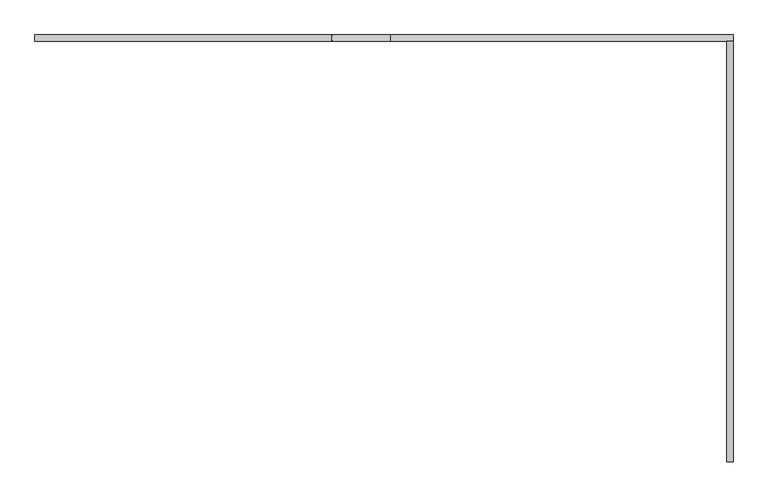
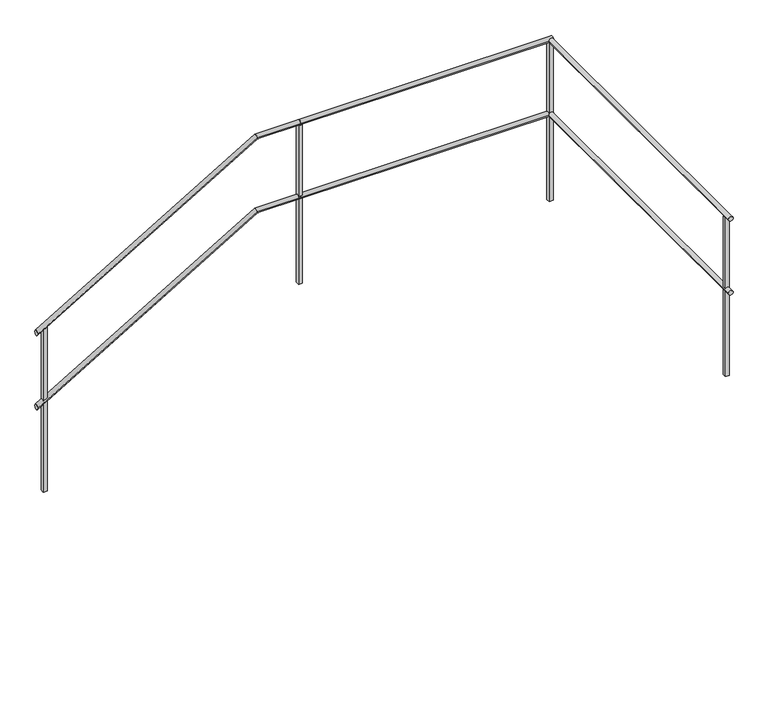
"""IFC4 building model written with IfcOpenShell, lengths in millimetres: railing geometry."""

from ifc_helpers import new_model, si_unit, frame, origin, place, context, project, spatial, polyline, circle_curve, ellipse_curve, outline, extrude, source, transform, mapped, element, save
from ifc_brep_helpers import plane_surface, cylinder_surface, advanced_brep


def railing_70c1d9d7(model_context):
    return source(origin(), model_context, "Body", "SolidModel", [
        advanced_brep(
        [(45466.7161135, 23749.5208589, 1584.9618634), (45496.7161135, 23749.5208589, 1584.9618634), (45466.7161135, 25734.1208589, 1584.9618634), (45496.7161135, 25734.1208589, 1584.9618634)],
        [
            (0, 1, circle_curve(frame((45481.7161135, 23749.5208589, 1584.9618634), z_axis=(0.0, -1.0, 0.0), x_axis=(1.0, 0.0, 0.0)), 15.0)),
            (1, 0, circle_curve(frame((45481.7161135, 23749.5208589, 1584.9618634), z_axis=(0.0, -1.0, 0.0), x_axis=(1.0, 0.0, 0.0)), 15.0)),
            (2, 3, circle_curve(frame((45481.7161135, 25734.1208589, 1584.9618634), z_axis=(0.0, 1.0, 0.0), x_axis=(1.0, 0.0, 0.0)), 15.0)),
            (3, 2, circle_curve(frame((45481.7161135, 25734.1208589, 1584.9618634), z_axis=(0.0, 1.0, 0.0), x_axis=(1.0, 0.0, 0.0)), 15.0)),
            (0, 2),
            (3, 1),
        ],
        [
            plane_surface(frame((45481.7161135, 23749.5208589, 1599.9618634), z_axis=(0.0, -1.0, 0.0), x_axis=(0.0, 0.0, 1.0))),
            plane_surface(frame((45481.7161135, 25734.1208589, 1599.9618634), z_axis=(0.0, 1.0, 0.0), x_axis=(0.0, 0.0, 1.0))),
            cylinder_surface(frame((45481.7161135, 23749.5208589, 1584.9618634), z_axis=(0.0, -1.0, 0.0), x_axis=(1.0, 0.0, 0.0)), 15.0),
        ],
        [
            (0, [[1, 2]]),
            (1, [[3, 4]]),
            (2, [[-1, 5, -4, 6]]),
            (2, [[-2, -6, -3, -5]]),
        ],
    ),
        advanced_brep(
        [(45496.7161135, 25734.1208589, 1584.9618634), (45496.7161135, 25764.1208589, 1584.9618634), (43882.1161135, 25734.1208589, 1584.9618634), (43882.1161135, 25764.1208589, 1584.9618634)],
        [
            (0, 1, circle_curve(frame((45496.7161135, 25749.1208589, 1584.9618634), z_axis=(1.0, 0.0, 0.0), x_axis=(0.0, 1.0, 0.0)), 15.0)),
            (1, 0, circle_curve(frame((45496.7161135, 25749.1208589, 1584.9618634), z_axis=(1.0, 0.0, 0.0), x_axis=(0.0, 1.0, 0.0)), 15.0)),
            (2, 3, circle_curve(frame((43882.1161135, 25749.1208589, 1584.9618634), z_axis=(-1.0, 0.0, 0.0), x_axis=(0.0, 1.0, 0.0)), 15.0)),
            (3, 2, circle_curve(frame((43882.1161135, 25749.1208589, 1584.9618634), z_axis=(-1.0, 0.0, 0.0), x_axis=(0.0, 1.0, 0.0)), 15.0)),
            (0, 2),
            (3, 1),
        ],
        [
            plane_surface(frame((45496.7161135, 25749.1208589, 1599.9618634), z_axis=(1.0, 0.0, 0.0), x_axis=(0.0, -1.0, 0.0))),
            plane_surface(frame((43882.1161135, 25749.1208589, 1599.9618634), z_axis=(-1.0, 0.0, 0.0), x_axis=(0.0, -1.0, 0.0))),
            cylinder_surface(frame((45496.7161135, 25749.1208589, 1584.9618634), z_axis=(1.0, 0.0, 0.0), x_axis=(0.0, 1.0, 0.0)), 15.0),
        ],
        [
            (0, [[1, 2]]),
            (1, [[3, 4]]),
            (2, [[-1, 5, -4, 6]]),
            (2, [[-2, -6, -3, -5]]),
        ],
    ),
        advanced_brep(
        [(43882.1161135, 25734.1208589, 1584.9618634), (43882.1161135, 25764.1208589, 1584.9618634), (43606.242552, 25734.1208589, 1584.9618634), (43606.242552, 25764.1208589, 1584.9618634), (42202.1161135, 25734.1208589, 749.1723166), (42202.1161135, 25764.1208589, 749.1723166)],
        [
            (0, 1, circle_curve(frame((43882.1161135, 25749.1208589, 1584.9618634), z_axis=(1.0, 0.0, 0.0), x_axis=(0.0, 1.0, 0.0)), 15.0)),
            (1, 0, circle_curve(frame((43882.1161135, 25749.1208589, 1584.9618634), z_axis=(1.0, 0.0, 0.0), x_axis=(0.0, 1.0, 0.0)), 15.0)),
            (0, 2),
            (2, 3, ellipse_curve(frame((43606.242552, 25749.1208589, 1584.9618634), z_axis=(0.9641817474962143, 0.0, 0.2652424509673111), x_axis=(0.265242450967311, 0.0, -0.9641817474962144)), 15.5572329, 15.0)),
            (3, 1),
            (3, 2, ellipse_curve(frame((43606.242552, 25749.1208589, 1584.9618634), z_axis=(0.9641817474962143, 0.0, 0.2652424509673111), x_axis=(0.265242450967311, 0.0, -0.9641817474962144)), 15.5572329, 15.0)),
            (4, 5, ellipse_curve(frame((42202.1161135, 25749.1208589, 749.1723166), z_axis=(-1.0, 0.0, 0.0), x_axis=(0.0, 0.0, 1.0)), 17.4562134, 15.0)),
            (5, 4, ellipse_curve(frame((42202.1161135, 25749.1208589, 749.1723166), z_axis=(-1.0, 0.0, 0.0), x_axis=(0.0, 0.0, 1.0)), 17.4562134, 15.0)),
            (2, 4),
            (5, 3),
        ],
        [
            plane_surface(frame((43882.1161135, 25749.1208589, 1599.9618634), z_axis=(1.0, 0.0, 0.0), x_axis=(0.0, -1.0, 0.0))),
            cylinder_surface(frame((43882.1161135, 25749.1208589, 1584.9618634), z_axis=(1.0, 0.0, 0.0), x_axis=(0.0, 1.0, 0.0)), 15.0),
            plane_surface(frame((42202.1161135, 25749.1208589, 766.62853), z_axis=(-1.0, 0.0, 0.0), x_axis=(0.0, -1.0, 0.0))),
            cylinder_surface(frame((43609.7883714, 25749.1208589, 1587.0724701), z_axis=(0.8592928844097072, 0.0, 0.5114838597676818), x_axis=(0.0, 1.0, 0.0)), 15.0),
        ],
        [
            (0, [[1, 2]]),
            (1, [[-1, 3, 4, 5]]),
            (1, [[-2, -5, 6, -3]]),
            (2, [[7, 8]]),
            (3, [[-4, 9, -8, 10]]),
            (3, [[-6, -10, -7, -9]]),
        ],
    ),
        advanced_brep(
        [(45466.7161135, 23749.5208589, 2084.9618634), (45496.7161135, 23749.5208589, 2084.9618634), (45466.7161135, 25734.1208589, 2084.9618634), (45496.7161135, 25734.1208589, 2084.9618634)],
        [
            (0, 1, circle_curve(frame((45481.7161135, 23749.5208589, 2084.9618634), z_axis=(0.0, -1.0, 0.0), x_axis=(1.0, 0.0, 0.0)), 15.0)),
            (1, 0, circle_curve(frame((45481.7161135, 23749.5208589, 2084.9618634), z_axis=(0.0, -1.0, 0.0), x_axis=(1.0, 0.0, 0.0)), 15.0)),
            (2, 3, circle_curve(frame((45481.7161135, 25734.1208589, 2084.9618634), z_axis=(0.0, 1.0, 0.0), x_axis=(1.0, 0.0, 0.0)), 15.0)),
            (3, 2, circle_curve(frame((45481.7161135, 25734.1208589, 2084.9618634), z_axis=(0.0, 1.0, 0.0), x_axis=(1.0, 0.0, 0.0)), 15.0)),
            (0, 2),
            (3, 1),
        ],
        [
            plane_surface(frame((45481.7161135, 23749.5208589, 2099.9618634), z_axis=(0.0, -1.0, 0.0), x_axis=(0.0, 0.0, 1.0))),
            plane_surface(frame((45481.7161135, 25734.1208589, 2099.9618634), z_axis=(0.0, 1.0, 0.0), x_axis=(0.0, 0.0, 1.0))),
            cylinder_surface(frame((45481.7161135, 23749.5208589, 2084.9618634), z_axis=(0.0, -1.0, 0.0), x_axis=(1.0, 0.0, 0.0)), 15.0),
        ],
        [
            (0, [[1, 2]]),
            (1, [[3, 4]]),
            (2, [[-1, 5, -4, 6]]),
            (2, [[-2, -6, -3, -5]]),
        ],
    ),
        advanced_brep(
        [(45496.7161135, 25734.1208589, 2084.9618634), (45496.7161135, 25764.1208589, 2084.9618634), (43882.1161135, 25734.1208589, 2084.9618634), (43882.1161135, 25764.1208589, 2084.9618634)],
        [
            (0, 1, circle_curve(frame((45496.7161135, 25749.1208589, 2084.9618634), z_axis=(1.0, 0.0, 0.0), x_axis=(0.0, 1.0, 0.0)), 15.0)),
            (1, 0, circle_curve(frame((45496.7161135, 25749.1208589, 2084.9618634), z_axis=(1.0, 0.0, 0.0), x_axis=(0.0, 1.0, 0.0)), 15.0)),
            (2, 3, circle_curve(frame((43882.1161135, 25749.1208589, 2084.9618634), z_axis=(-1.0, 0.0, 0.0), x_axis=(0.0, 1.0, 0.0)), 15.0)),
            (3, 2, circle_curve(frame((43882.1161135, 25749.1208589, 2084.9618634), z_axis=(-1.0, 0.0, 0.0), x_axis=(0.0, 1.0, 0.0)), 15.0)),
            (0, 2),
            (3, 1),
        ],
        [
            plane_surface(frame((45496.7161135, 25749.1208589, 2099.9618634), z_axis=(1.0, 0.0, 0.0), x_axis=(0.0, -1.0, 0.0))),
            plane_surface(frame((43882.1161135, 25749.1208589, 2099.9618634), z_axis=(-1.0, 0.0, 0.0), x_axis=(0.0, -1.0, 0.0))),
            cylinder_surface(frame((45496.7161135, 25749.1208589, 2084.9618634), z_axis=(1.0, 0.0, 0.0), x_axis=(0.0, 1.0, 0.0)), 15.0),
        ],
        [
            (0, [[1, 2]]),
            (1, [[3, 4]]),
            (2, [[-1, 5, -4, 6]]),
            (2, [[-2, -6, -3, -5]]),
        ],
    ),
        advanced_brep(
        [(43882.1161135, 25734.1208589, 2084.9618634), (43882.1161135, 25764.1208589, 2084.9618634), (43606.242552, 25734.1208589, 2084.9618634), (43606.242552, 25764.1208589, 2084.9618634), (42202.1161135, 25734.1208589, 1249.1723166), (42202.1161135, 25764.1208589, 1249.1723166)],
        [
            (0, 1, circle_curve(frame((43882.1161135, 25749.1208589, 2084.9618634), z_axis=(1.0, 0.0, 0.0), x_axis=(0.0, 1.0, 0.0)), 15.0)),
            (1, 0, circle_curve(frame((43882.1161135, 25749.1208589, 2084.9618634), z_axis=(1.0, 0.0, 0.0), x_axis=(0.0, 1.0, 0.0)), 15.0)),
            (0, 2),
            (2, 3, ellipse_curve(frame((43606.242552, 25749.1208589, 2084.9618634), z_axis=(0.9641817474962143, 0.0, 0.2652424509673111), x_axis=(0.265242450967311, 0.0, -0.9641817474962144)), 15.5572329, 15.0)),
            (3, 1),
            (3, 2, ellipse_curve(frame((43606.242552, 25749.1208589, 2084.9618634), z_axis=(0.9641817474962143, 0.0, 0.2652424509673111), x_axis=(0.265242450967311, 0.0, -0.9641817474962144)), 15.5572329, 15.0)),
            (4, 5, ellipse_curve(frame((42202.1161135, 25749.1208589, 1249.1723166), z_axis=(-1.0, 0.0, 0.0), x_axis=(0.0, 0.0, 1.0)), 17.4562134, 15.0)),
            (5, 4, ellipse_curve(frame((42202.1161135, 25749.1208589, 1249.1723166), z_axis=(-1.0, 0.0, 0.0), x_axis=(0.0, 0.0, 1.0)), 17.4562134, 15.0)),
            (2, 4),
            (5, 3),
        ],
        [
            plane_surface(frame((43882.1161135, 25749.1208589, 2099.9618634), z_axis=(1.0, 0.0, 0.0), x_axis=(0.0, -1.0, 0.0))),
            cylinder_surface(frame((43882.1161135, 25749.1208589, 2084.9618634), z_axis=(1.0, 0.0, 0.0), x_axis=(0.0, 1.0, 0.0)), 15.0),
            plane_surface(frame((42202.1161135, 25749.1208589, 1266.62853), z_axis=(-1.0, 0.0, 0.0), x_axis=(0.0, -1.0, 0.0))),
            cylinder_surface(frame((43609.7883714, 25749.1208589, 2087.0724701), z_axis=(0.8592928844097072, 0.0, 0.5114838597676818), x_axis=(0.0, 1.0, 0.0)), 15.0),
        ],
        [
            (0, [[1, 2]]),
            (1, [[-1, 3, 4, 5]]),
            (1, [[-2, -5, 6, -3]]),
            (2, [[7, 8]]),
            (3, [[-4, 9, -8, 10]]),
            (3, [[-6, -10, -7, -9]]),
        ],
    ),
        extrude(outline(polyline([(43894.6161135, 25761.6208589), (43894.6161135, 25736.6208589), (43869.6161135, 25736.6208589), (43869.6161135, 25761.6208589), (43894.6161135, 25761.6208589)])), frame((0.0, 0.0, 999.9618634), z_axis=(0.0, 0.0, 1.0), x_axis=(1.0, 0.0, 0.0)), (0.0, 0.0, 1.0), 1070.0),
        extrude(outline(polyline([(45494.2161135, 25736.6208589), (45469.2161135, 25736.6208589), (45469.2161135, 25761.6208589), (45494.2161135, 25761.6208589), (45494.2161135, 25736.6208589)])), frame((0.0, 0.0, 999.9618634), z_axis=(0.0, 0.0, 1.0), x_axis=(1.0, 0.0, 0.0)), (0.0, 0.0, 1.0), 1070.0),
        extrude(outline(polyline([(166.62853, 42264.6161135), (1273.830911, 42264.6161135), (1258.9499586, 42239.6161135), (166.62853, 42239.6161135), (166.62853, 42264.6161135)])), frame((0.0, 25736.6208589, 0.0), z_axis=(0.0, 1.0, 0.0), x_axis=(0.0, 0.0, 1.0)), (0.0, 0.0, 1.0), 25.0),
        extrude(outline(polyline([(45494.2161135, 23787.0208589), (45469.2161135, 23787.0208589), (45469.2161135, 23812.0208589), (45494.2161135, 23812.0208589), (45494.2161135, 23787.0208589)])), frame((0.0, 0.0, 999.9618634), z_axis=(0.0, 0.0, 1.0), x_axis=(1.0, 0.0, 0.0)), (0.0, 0.0, 1.0), 1070.0),
    ])


if __name__ == "__main__":
    model = new_model("IFC4")
    model_context = context("Model", 3, world=origin())
    ifc_project = project(units=[si_unit("LENGTHUNIT", "METRE", prefix="MILLI")], contexts=[model_context])
    site = spatial("IfcSite", under=ifc_project)
    building = spatial("IfcBuilding", under=site)
    placement = place(None, origin())
    railing_shape = railing_70c1d9d7(model_context)
    element("IfcRailing", 1, at=placement, inside=building, context=model_context, shape_type="MappedRepresentation", body=[
        mapped(railing_shape, transform((0.0, 0.0, 0.0), x_axis=(1.0, 0.0, 0.0), y_axis=(0.0, 1.0, 0.0), z_axis=(0.0, 0.0, 1.0))),
    ])
    save(model, "model.ifc")
